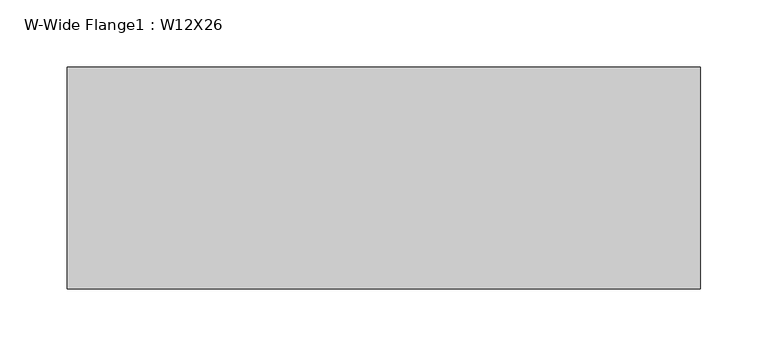
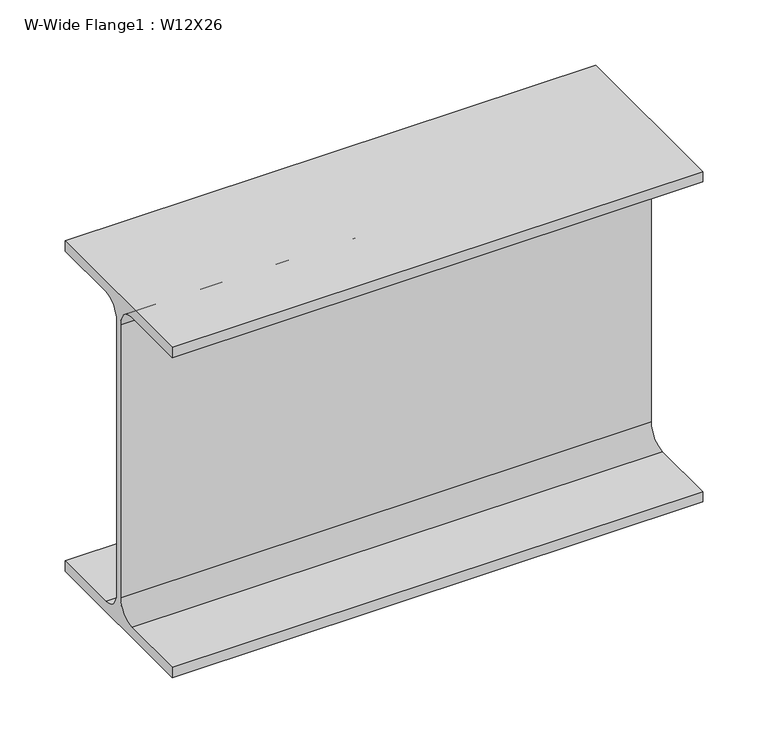
"""IFC4 building model written with IfcOpenShell, lengths in millimetres: beam geometry, W-Wide Flange1 : W12X26."""

from ifc_helpers import new_model, si_unit, point, frame, frame_2d, origin, place, context, project, spatial, polyline, circle_curve, trimmed, segment, composite_curve, outline, extrude, source, transform, mapped, element, save


def w_wide_flange1_w12x26_54103811(model_context):
    return source(origin(), model_context, "Body", "SweptSolid", [
        extrude(outline(composite_curve([segment(polyline([(82.423, -145.288), (82.423, -154.94), (-82.423, -154.94), (-82.423, -145.288), (-20.2565, -145.288)]), True, "CONTINUOUS"), segment(trimmed(circle_curve(frame_2d((-20.2565, -127.9525)), 17.3355), [point((-20.2565, -145.288))], [point((-2.921, -127.9525))], True, "CARTESIAN"), True, "CONTINUOUS"), segment(polyline([(-2.921, -127.9525), (-2.921, 127.9525)]), True, "CONTINUOUS"), segment(trimmed(circle_curve(frame_2d((-20.2565, 127.9525)), 17.3355), [point((-2.921, 127.9525))], [point((-20.2565, 145.288))], True, "CARTESIAN"), True, "CONTINUOUS"), segment(polyline([(-20.2565, 145.288), (-82.423, 145.288), (-82.423, 154.94), (82.423, 154.94), (82.423, 145.288), (20.2565, 145.288)]), True, "CONTINUOUS"), segment(trimmed(circle_curve(frame_2d((20.2565, 127.9525)), 17.3355), [point((20.2565, 145.288))], [point((2.921, 127.9525))], True, "CARTESIAN"), True, "CONTINUOUS"), segment(polyline([(2.921, 127.9525), (2.921, -127.9525)]), True, "CONTINUOUS"), segment(trimmed(circle_curve(frame_2d((20.2565, -127.9525)), 17.3355), [point((2.921, -127.9525))], [point((20.2565, -145.288))], True, "CARTESIAN"), True, "CONTINUOUS"), segment(polyline([(20.2565, -145.288), (82.423, -145.288)]), True, "CONTINUOUS")], self_intersect=False)), frame((-180.5371134, 0.0, 0.0), z_axis=(1.0, 0.0, 0.0), x_axis=(0.0, 1.0, 0.0)), (0.0, 0.0, 1.0), 470.7668191),
    ])


if __name__ == "__main__":
    model = new_model("IFC4")
    model_context = context("Model", 3, world=origin())
    ifc_project = project(units=[si_unit("LENGTHUNIT", "METRE", prefix="MILLI")], contexts=[model_context])
    site = spatial("IfcSite", under=ifc_project)
    building = spatial("IfcBuilding", under=site)
    placement = place(None, origin())
    w_wide_flange1_w12x26_shape = w_wide_flange1_w12x26_54103811(model_context)
    element("IfcBeam", 1, ObjectType="W-Wide Flange1 : W12X26", at=placement, inside=building, context=model_context, shape_type="MappedRepresentation", body=[
        mapped(w_wide_flange1_w12x26_shape, transform((0.0, 0.0, 0.0), x_axis=(1.0, 0.0, 0.0), y_axis=(0.0, 1.0, 0.0), z_axis=(0.0, 0.0, 1.0))),
    ])
    save(model, "model.ifc")

# Revit data of these elements
# Type "W-Wide Flange1 : W12X26"
#   Assembly Code = "B10"
#   W = 26
#   Start Extension Calculation [instance default] = 10' - 0"
#   Start Extension [instance default] = -0' - 0 1/2"
#   End Extension Calculation [instance default] = 10' - 0"
#   End Extension [instance default] = -0' - 0 1/2"
#   Length [instance default] = 5' - 0"
#   bf = 0' - 6.49"
#   d = 1' - 0.2"
#   k = 0' - 1 1/16"
#   k2 = 0' - 0.6825"
#   tf = 0' - 0.38"
#   tw = 0' - 0.23"
#   A = 0.053125 SF
#   Structural Material [instance default] = Metal - Steel - ASTM A992
# Element 1 (IfcBeam, "W-Wide Flange1 : W12X26")
#   Materials on its faces: "Metal - Steel - ASTM A992"
# Materials
#   "Metal - Steel - ASTM A992": class "Metal", colour RGB 199 199 199, transparency 0
